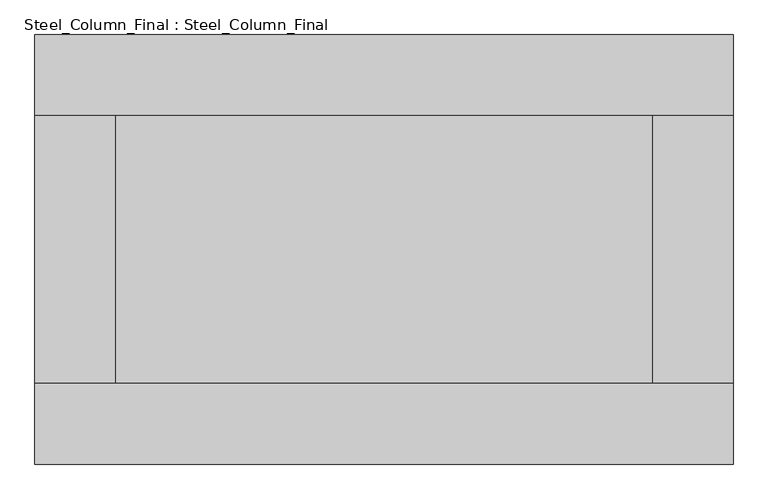
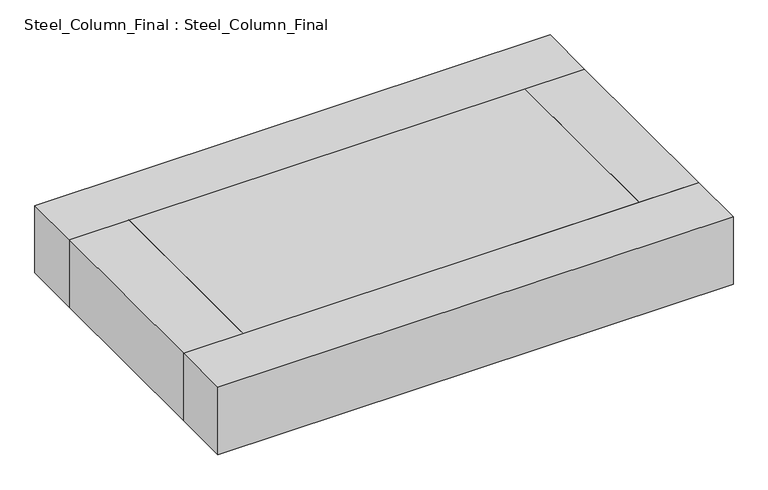
"""IFC4 building model written with IfcOpenShell, lengths in millimetres: proxy geometry, Steel_Column_Final : Steel_Column_Final."""

from ifc_helpers import new_model, si_unit, frame, origin, place, context, project, spatial, polyline, outline, extrude, source, transform, mapped, element, save


def steel_column_final_steel_column_final_5a21aa61(model_context):
    return source(origin(), model_context, "Body", "SweptSolid", [
        extrude(outline(polyline([(6500.0, 2500.0), (-6500.0, 2500.0), (-6500.0, 4000.0), (6500.0, 4000.0), (6500.0, 2500.0)])), frame((0.0, 0.0, 106900.0), z_axis=(0.0, 0.0, 1.0), x_axis=(1.0, 0.0, 0.0)), (0.0, 0.0, 1.0), 1800.0),
        extrude(outline(polyline([(-6500.0, -2500.0), (6500.0, -2500.0), (6500.0, -4000.0), (-6500.0, -4000.0), (-6500.0, -2500.0)])), frame((0.0, 0.0, 106900.0), z_axis=(0.0, 0.0, 1.0), x_axis=(1.0, 0.0, 0.0)), (0.0, 0.0, 1.0), 1800.0),
        extrude(outline(polyline([(5000.0, -2500.0), (5000.0, 2500.0), (6500.0, 2500.0), (6500.0, -2500.0), (5000.0, -2500.0)])), frame((0.0, 0.0, 106900.0), z_axis=(0.0, 0.0, 1.0), x_axis=(1.0, 0.0, 0.0)), (0.0, 0.0, 1.0), 1800.0),
        extrude(outline(polyline([(-5000.0, 2500.0), (-5000.0, -2500.0), (-6500.0, -2500.0), (-6500.0, 2500.0), (-5000.0, 2500.0)])), frame((0.0, 0.0, 106900.0), z_axis=(0.0, 0.0, 1.0), x_axis=(1.0, 0.0, 0.0)), (0.0, 0.0, 1.0), 1800.0),
        extrude(outline(polyline([(-5000.0, -2500.0), (-5000.0, 2500.0), (5000.0, 2500.0), (5000.0, -2500.0), (-5000.0, -2500.0)])), frame((0.0, 0.0, 106900.0), z_axis=(0.0, 0.0, 1.0), x_axis=(1.0, 0.0, 0.0)), (0.0, 0.0, 1.0), 1800.0),
    ])


if __name__ == "__main__":
    model = new_model("IFC4")
    model_context = context("Model", 3, world=origin())
    ifc_project = project(units=[si_unit("LENGTHUNIT", "METRE", prefix="MILLI")], contexts=[model_context])
    site = spatial("IfcSite", under=ifc_project)
    building = spatial("IfcBuilding", under=site)
    placement = place(None, origin())
    steel_column_final_steel_column_final_shape = steel_column_final_steel_column_final_5a21aa61(model_context)
    element("IfcBuildingElementProxy", 1, Name="Steel_Column_Final : Steel_Column_Final", ObjectType="Steel_Column_Final : Steel_Column_Final", at=placement, inside=building, context=model_context, shape_type="MappedRepresentation", body=[
        mapped(steel_column_final_steel_column_final_shape, transform((0.0, 0.0, 0.0), x_axis=(1.0, 0.0, 0.0), y_axis=(0.0, 1.0, 0.0), z_axis=(0.0, 0.0, 1.0))),
    ])
    save(model, "model.ifc")

# Revit data of these elements
# Type "Steel_Column_Final : Steel_Column_Final"
#   Top Width [instance default] = 5000 mm
#   Top Length = 10000 mm
#   Length = 21000 mm
#   Height [instance default] = 50000 mm
#   Bottom Width [instance default] = 5000 mm
#   Default Elevation = 0
# Element 1 (IfcBuildingElementProxy, "Steel_Column_Final : Steel_Column_Final")
#   Height = 106900 mm
